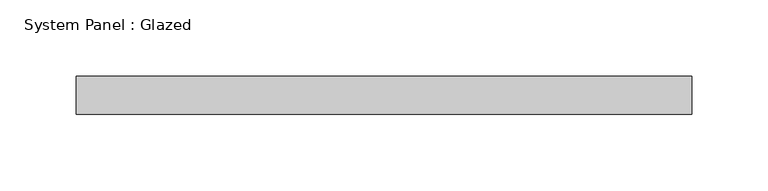
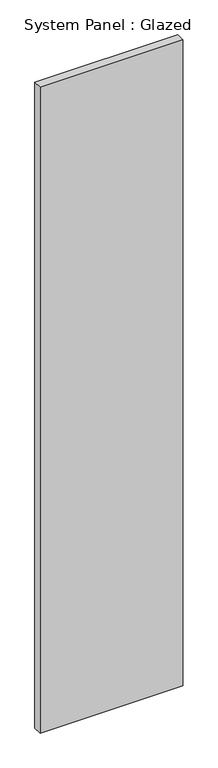
"""IFC4 building model written with IfcOpenShell, lengths in millimetres: plate geometry, System Panel : Glazed."""

import ifcopenshell
import ifcopenshell.guid

model = None  # the IFC model being written
_history = None  # IfcOwnerHistory: only IFC2X3 demands one
_inside = {}  # id of a spatial element -> (the spatial element, [elements in it])
_under = {}  # id of a project, library or spatial element -> (it, [spatial elements below it])
_declared = {}  # id of a project -> (the project, [libraries it declares])
_typed = {}  # id of a type object -> (the type object, [elements of that type])
_made_of = {}  # id of a material, layer set ... -> (it, [elements and type objects made of it])


def new_model(schema):
    """Start an empty IFC model of exactly this schema.

    Asked for "IFC4X3", IfcOpenShell would pick the latest addendum, in which some entities
    have other attributes; the version numbers below select the first issue.
    IFC2X3 requires an IfcOwnerHistory on every rooted entity: one is made here for all.
    """
    global model, _history
    if schema == "IFC4X3":
        model = ifcopenshell.file(schema_version=(4, 3, 0, 0))
    else:
        model = ifcopenshell.file(schema=schema)
    _inside.clear()
    _under.clear()
    _declared.clear()
    _typed.clear()
    _made_of.clear()
    _history = None
    if model.schema == "IFC2X3":
        org = make("IfcOrganization", Name="unknown")
        user = make(
            "IfcPersonAndOrganization",
            ThePerson=make("IfcPerson", FamilyName="unknown"),
            TheOrganization=org,
        )
        app = make(
            "IfcApplication",
            ApplicationDeveloper=org,
            Version="unknown",
            ApplicationFullName="unknown",
            ApplicationIdentifier="unknown",
        )
        _history = make(
            "IfcOwnerHistory",
            OwningUser=user,
            OwningApplication=app,
            ChangeAction="ADDED",
            CreationDate=0,
        )
    return model


def make(cls, **values):
    """One entity of the class cls with the attributes given. An attribute that is None is left unset."""
    return model.create_entity(
        cls, **{name: value for name, value in values.items() if value is not None}
    )


def rooted(cls, **values):
    """An entity with a GlobalId (a new one), such as an element, a storey or a relation."""
    return make(cls, GlobalId=ifcopenshell.guid.new(), OwnerHistory=_history, **values)


def si_unit(unit_type, name, prefix=None):
    """IfcSIUnit, for example si_unit("LENGTHUNIT", "METRE", prefix="MILLI")."""
    return make("IfcSIUnit", UnitType=unit_type, Prefix=prefix, Name=name)


def assignment(units):
    """IfcUnitAssignment: the units of a project."""
    return None if units is None else make("IfcUnitAssignment", Units=units)


def point(xyz):
    """IfcCartesianPoint."""
    return None if xyz is None else make("IfcCartesianPoint", Coordinates=xyz)


def direction(xyz):
    """IfcDirection."""
    return None if xyz is None else make("IfcDirection", DirectionRatios=xyz)


def frame(location, z_axis=None, x_axis=None):
    """IfcAxis2Placement3D, a coordinate frame: its origin and axes. An axis left out is left unset."""
    return make(
        "IfcAxis2Placement3D",
        Location=point(location),
        Axis=direction(z_axis),
        RefDirection=direction(x_axis),
    )


def origin():
    """The frame at (0, 0, 0) with its axes left unset."""
    return frame((0.0, 0.0, 0.0))


def origin_with_axes():
    """The frame at (0, 0, 0) with the z axis (0, 0, 1) and the x axis (1, 0, 0) written out."""
    return frame((0.0, 0.0, 0.0), z_axis=(0.0, 0.0, 1.0), x_axis=(1.0, 0.0, 0.0))


def place(relative_to, where):
    """IfcLocalPlacement: puts the frame where relative to a parent placement (None: the world)."""
    return make(
        "IfcLocalPlacement", PlacementRelTo=relative_to, RelativePlacement=where
    )


def context(
    kind, dimensions, precision=None, world=None, true_north=None, identifier=None
):
    """IfcGeometricRepresentationContext, for example the 3D "Model" context."""
    return make(
        "IfcGeometricRepresentationContext",
        ContextIdentifier=identifier,
        ContextType=kind,
        CoordinateSpaceDimension=dimensions,
        Precision=precision,
        WorldCoordinateSystem=world,
        TrueNorth=true_north,
    )


def project(units=None, contexts=None):
    """IfcProject with its units and contexts."""
    return rooted(
        "IfcProject",
        Name="project",
        RepresentationContexts=contexts,
        UnitsInContext=assignment(units),
    )


def spatial(cls, under=None, at=None, **own):
    """A site, building, storey or space (cls), placed at a placement, below another one or the project."""
    s = rooted(cls, ObjectPlacement=at, **own)
    if under is not None:
        _under.setdefault(under.id(), (under, []))[1].append(s)
    return s


def polyline(points):
    """IfcPolyline through the points."""
    return make("IfcPolyline", Points=[point(p) for p in points])


def outline(outer, holes=None, kind="AREA"):
    """IfcArbitraryClosedProfileDef: a profile drawn as a closed curve; with holes, ...WithVoids."""
    if holes is None:
        return make("IfcArbitraryClosedProfileDef", ProfileType=kind, OuterCurve=outer)
    return make(
        "IfcArbitraryProfileDefWithVoids",
        ProfileType=kind,
        OuterCurve=outer,
        InnerCurves=holes,
    )


def extrude(swept, where, along, depth):
    """IfcExtrudedAreaSolid: the profile swept, set in the frame where, extruded along a direction by depth."""
    return make(
        "IfcExtrudedAreaSolid",
        SweptArea=swept,
        Position=where,
        ExtrudedDirection=direction(along),
        Depth=depth,
    )


def shape(context_of_items, identifier, shape_type, items):
    """IfcShapeRepresentation: the items that make up one representation, for example the "Body"."""
    return make(
        "IfcShapeRepresentation",
        ContextOfItems=context_of_items,
        RepresentationIdentifier=identifier,
        RepresentationType=shape_type,
        Items=items,
    )


def source(mapping_origin, context_of_items, identifier, shape_type, items):
    """IfcRepresentationMap: a shape defined once, which mapped items show again and again."""
    return make(
        "IfcRepresentationMap",
        MappingOrigin=mapping_origin,
        MappedRepresentation=shape(context_of_items, identifier, shape_type, items),
    )


def transform(
    local_origin,
    x_axis=None,
    y_axis=None,
    z_axis=None,
    scale=None,
    scale2=None,
    scale3=None,
    uniform=True,
):
    """IfcCartesianTransformationOperator3D, or its non-uniform kind. x_axis, y_axis, z_axis: its Axis1, 2, 3."""
    if uniform:
        return make(
            "IfcCartesianTransformationOperator3D",
            Axis1=direction(x_axis),
            Axis2=direction(y_axis),
            LocalOrigin=point(local_origin),
            Scale=scale,
            Axis3=direction(z_axis),
        )
    return make(
        "IfcCartesianTransformationOperator3DnonUniform",
        Axis1=direction(x_axis),
        Axis2=direction(y_axis),
        LocalOrigin=point(local_origin),
        Scale=scale,
        Axis3=direction(z_axis),
        Scale2=scale2,
        Scale3=scale3,
    )


def mapped(mapping_source, mapping_target):
    """IfcMappedItem: shows the shape of a source again, moved by a transform."""
    return make(
        "IfcMappedItem", MappingSource=mapping_source, MappingTarget=mapping_target
    )


def made_of(thing, what):
    """Note that an element or type object is made of a material, layer set ...; save() writes the relation."""
    if what is not None:
        _made_of.setdefault(what.id(), (what, []))[1].append(thing)
    return thing


def element(
    cls,
    number,
    at=None,
    inside=None,
    cuts=None,
    type_object=None,
    material=None,
    context=None,
    identifier="Body",
    shape_type=None,
    held_by="IfcProductDefinitionShape",
    body=None,
    shapes=None,
    **own,
):
    """One element of the class cls, such as IfcWall. Its Tag is "e" and its number.

    at: its placement. inside: the storey or other place that contains it. cuts: it is an
    opening in that element (IfcRelVoidsElement). A single representation is given by context,
    identifier, shape_type and body (its items); several are given by shapes. held_by: the class
    of the entity that holds the representations. save() writes the other relations.
    """
    e = rooted(cls, Tag="e%d" % number, ObjectPlacement=at, **own)
    if body is not None:
        shapes = [shape(context, identifier, shape_type, body)]
    if shapes is not None:
        e.Representation = make(held_by, Representations=shapes)
    if inside is not None:
        _inside.setdefault(inside.id(), (inside, []))[1].append(e)
    if cuts is not None:
        rooted(
            "IfcRelVoidsElement", RelatingBuildingElement=cuts, RelatedOpeningElement=e
        )
    if type_object is not None:
        _typed.setdefault(type_object.id(), (type_object, []))[1].append(e)
    return made_of(e, material)


def aggregate(whole, parts):
    """IfcRelAggregates: a whole, such as a stair, and the parts it consists of."""
    return rooted("IfcRelAggregates", RelatingObject=whole, RelatedObjects=parts)


def save(model, path):
    """Write the relations noted so far, then the file.

    IfcRelAggregates (storeys below a building ...), IfcRelContainedInSpatialStructure (elements
    in a storey), IfcRelDefinesByType, IfcRelAssociatesMaterial and IfcRelDeclares: one each for
    every whole, place, type object, material and project.
    """
    for whole, parts in _under.values():
        aggregate(whole, parts)
    for where, things in _inside.values():
        rooted(
            "IfcRelContainedInSpatialStructure",
            RelatedElements=things,
            RelatingStructure=where,
        )
    for kind, things in _typed.values():
        rooted("IfcRelDefinesByType", RelatedObjects=things, RelatingType=kind)
    for what, things in _made_of.values():
        rooted("IfcRelAssociatesMaterial", RelatedObjects=things, RelatingMaterial=what)
    for by, libraries in _declared.values():
        rooted("IfcRelDeclares", RelatingContext=by, RelatedDefinitions=libraries)
    model.write(path)


def system_panel_glazed_06eb0cda(model_context):
    return source(origin(), model_context, "Body", "SweptSolid", [
        extrude(outline(polyline([(202.4999999, 24.5), (-202.4999999, 24.5), (-202.4999999, 49.5), (202.4999999, 49.5), (202.4999999, 24.5)])), origin_with_axes(), (0.0, 0.0, 1.0), 1934.1016494),
    ])


if __name__ == "__main__":
    model = new_model("IFC4")
    model_context = context("Model", 3, world=origin())
    ifc_project = project(units=[si_unit("LENGTHUNIT", "METRE", prefix="MILLI")], contexts=[model_context])
    site = spatial("IfcSite", under=ifc_project)
    building = spatial("IfcBuilding", under=site)
    placement = place(None, origin())
    system_panel_glazed_shape = system_panel_glazed_06eb0cda(model_context)
    element("IfcPlate", 1, ObjectType="System Panel : Glazed", at=placement, inside=building, context=model_context, shape_type="MappedRepresentation", body=[
        mapped(system_panel_glazed_shape, transform((0.0, 0.0, 0.0), x_axis=(1.0, 0.0, 0.0), y_axis=(0.0, 1.0, 0.0), z_axis=(0.0, 0.0, 1.0))),
    ])
    save(model, "model.ifc")

# Revit data of these elements
# Type "System Panel : Glazed"
#   Keynote = "H11"
#   Construction Type Id = "GSP4R"
#   Analytic Construction = "1/8 in Pilkington single glazing"
#   Visual Light Transmittance = 0.9
#   Solar Heat Gain Coefficient = 0.86
#   Heat Transfer Coefficient (U) = 6.7069 W/(m²·K)
#   Define Thermal Properties by = 1
# Element 1 (IfcPlate, "System Panel : Glazed")
#   Materials on its faces: "Glass"
# Materials
#   "Glass": class "Glass", colour RGB 0 128 192, transparency 0.9, Description = "Soda Lime Glass", Cost = 0
